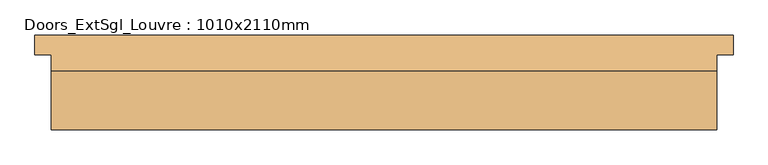
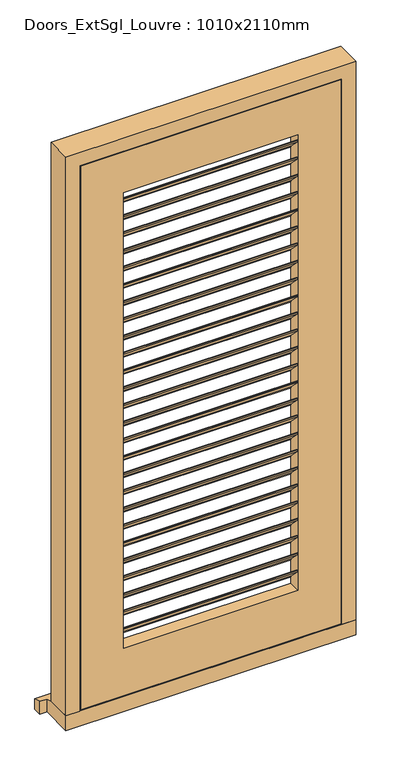
"""IFC4 building model written with IfcOpenShell, lengths in millimetres: door geometry, Doors_ExtSgl_Louvre : 1010x2110mm."""

from ifc_helpers import new_model, si_unit, point, frame, frame_2d, origin, place, context, project, spatial, polyline, circle_curve, trimmed, segment, composite_curve, outline, extrude, faceted_brep, source, transform, mapped, element, save


def doors_extsgl_louvre_1010x2110mm_50524d4c(model_context):
    return source(origin(), model_context, "Body", "SolidModel", [
        extrude(outline(composite_curve([segment(trimmed(circle_curve(frame_2d((1200.0, -378.5)), 19.0), [point((1200.0, -359.5))], [point((1200.0, -397.5))], False, "CARTESIAN"), True, "CONTINUOUS"), segment(trimmed(circle_curve(frame_2d((1200.0, -378.5)), 19.0), [point((1200.0, -397.5))], [point((1200.0, -359.5))], False, "CARTESIAN"), True, "CONTINUOUS")], self_intersect=False), holes=[composite_curve([segment(polyline([(1197.6985978, -377.5235023), (1188.3126735, -377.5235023), (1188.3126735, -379.4936963), (1197.7059713, -379.4936963)]), True, "CONTINUOUS"), segment(trimmed(circle_curve(frame_2d((1200.0, -378.5)), 2.5), [point((1197.7059713, -379.4936963))], [point((1197.6985978, -377.5235023))], True, "CARTESIAN"), True, "CONTINUOUS")], self_intersect=False)]), frame((0.0, 96.25, 0.0), z_axis=(0.0, 1.0, 0.0), x_axis=(0.0, 0.0, 1.0)), (0.0, 0.0, 1.0), 3.0),
        extrude(outline(polyline([(56.25, 1821.22), (96.25, 1781.22), (96.25, 1777.22), (93.25, 1777.22), (93.25, 1779.9773593), (53.25, 1819.9773593), (53.25, 1825.22), (56.25, 1825.22), (56.25, 1821.22)])), frame((-303.5, 0.0, 0.0), z_axis=(1.0, 0.0, 0.0), x_axis=(0.0, 1.0, 0.0)), (0.0, 0.0, 1.0), 607.0),
        extrude(outline(polyline([(56.25, 1757.94), (96.25, 1717.94), (96.25, 1713.94), (93.25, 1713.94), (93.25, 1716.6973593), (53.25, 1756.6973593), (53.25, 1761.94), (56.25, 1761.94), (56.25, 1757.94)])), frame((-303.5, 0.0, 0.0), z_axis=(1.0, 0.0, 0.0), x_axis=(0.0, 1.0, 0.0)), (0.0, 0.0, 1.0), 607.0),
        extrude(outline(polyline([(56.25, 1694.66), (96.25, 1654.66), (96.25, 1650.66), (93.25, 1650.66), (93.25, 1653.4173593), (53.25, 1693.4173593), (53.25, 1698.66), (56.25, 1698.66), (56.25, 1694.66)])), frame((-303.5, 0.0, 0.0), z_axis=(1.0, 0.0, 0.0), x_axis=(0.0, 1.0, 0.0)), (0.0, 0.0, 1.0), 607.0),
        extrude(outline(polyline([(56.25, 1631.38), (96.25, 1591.38), (96.25, 1587.38), (93.25, 1587.38), (93.25, 1590.1373593), (53.25, 1630.1373593), (53.25, 1635.38), (56.25, 1635.38), (56.25, 1631.38)])), frame((-303.5, 0.0, 0.0), z_axis=(1.0, 0.0, 0.0), x_axis=(0.0, 1.0, 0.0)), (0.0, 0.0, 1.0), 607.0),
        extrude(outline(polyline([(56.25, 1568.1), (96.25, 1528.1), (96.25, 1524.1), (93.25, 1524.1), (93.25, 1526.8573593), (53.25, 1566.8573593), (53.25, 1572.1), (56.25, 1572.1), (56.25, 1568.1)])), frame((-303.5, 0.0, 0.0), z_axis=(1.0, 0.0, 0.0), x_axis=(0.0, 1.0, 0.0)), (0.0, 0.0, 1.0), 607.0),
        extrude(outline(polyline([(56.25, 1504.82), (96.25, 1464.82), (96.25, 1460.82), (93.25, 1460.82), (93.25, 1463.5773593), (53.25, 1503.5773593), (53.25, 1508.82), (56.25, 1508.82), (56.25, 1504.82)])), frame((-303.5, 0.0, 0.0), z_axis=(1.0, 0.0, 0.0), x_axis=(0.0, 1.0, 0.0)), (0.0, 0.0, 1.0), 607.0),
        extrude(outline(polyline([(56.25, 1441.54), (96.25, 1401.54), (96.25, 1397.54), (93.25, 1397.54), (93.25, 1400.2973593), (53.25, 1440.2973593), (53.25, 1445.54), (56.25, 1445.54), (56.25, 1441.54)])), frame((-303.5, 0.0, 0.0), z_axis=(1.0, 0.0, 0.0), x_axis=(0.0, 1.0, 0.0)), (0.0, 0.0, 1.0), 607.0),
        extrude(outline(polyline([(56.25, 1378.26), (96.25, 1338.26), (96.25, 1334.26), (93.25, 1334.26), (93.25, 1337.0173593), (53.25, 1377.0173593), (53.25, 1382.26), (56.25, 1382.26), (56.25, 1378.26)])), frame((-303.5, 0.0, 0.0), z_axis=(1.0, 0.0, 0.0), x_axis=(0.0, 1.0, 0.0)), (0.0, 0.0, 1.0), 607.0),
        extrude(outline(polyline([(56.25, 1314.98), (96.25, 1274.98), (96.25, 1270.98), (93.25, 1270.98), (93.25, 1273.7373593), (53.25, 1313.7373593), (53.25, 1318.98), (56.25, 1318.98), (56.25, 1314.98)])), frame((-303.5, 0.0, 0.0), z_axis=(1.0, 0.0, 0.0), x_axis=(0.0, 1.0, 0.0)), (0.0, 0.0, 1.0), 607.0),
        extrude(outline(polyline([(56.25, 1251.7), (96.25, 1211.7), (96.25, 1207.7), (93.25, 1207.7), (93.25, 1210.4573593), (53.25, 1250.4573593), (53.25, 1255.7), (56.25, 1255.7), (56.25, 1251.7)])), frame((-303.5, 0.0, 0.0), z_axis=(1.0, 0.0, 0.0), x_axis=(0.0, 1.0, 0.0)), (0.0, 0.0, 1.0), 607.0),
        extrude(outline(polyline([(56.25, 1188.42), (96.25, 1148.42), (96.25, 1144.42), (93.25, 1144.42), (93.25, 1147.1773593), (53.25, 1187.1773593), (53.25, 1192.42), (56.25, 1192.42), (56.25, 1188.42)])), frame((-303.5, 0.0, 0.0), z_axis=(1.0, 0.0, 0.0), x_axis=(0.0, 1.0, 0.0)), (0.0, 0.0, 1.0), 607.0),
        extrude(outline(polyline([(56.25, 1125.14), (96.25, 1085.14), (96.25, 1081.14), (93.25, 1081.14), (93.25, 1083.8973593), (53.25, 1123.8973593), (53.25, 1129.14), (56.25, 1129.14), (56.25, 1125.14)])), frame((-303.5, 0.0, 0.0), z_axis=(1.0, 0.0, 0.0), x_axis=(0.0, 1.0, 0.0)), (0.0, 0.0, 1.0), 607.0),
        extrude(outline(polyline([(56.25, 1061.86), (96.25, 1021.86), (96.25, 1017.86), (93.25, 1017.86), (93.25, 1020.6173593), (53.25, 1060.6173593), (53.25, 1065.86), (56.25, 1065.86), (56.25, 1061.86)])), frame((-303.5, 0.0, 0.0), z_axis=(1.0, 0.0, 0.0), x_axis=(0.0, 1.0, 0.0)), (0.0, 0.0, 1.0), 607.0),
        extrude(outline(polyline([(56.25, 998.58), (96.25, 958.58), (96.25, 954.58), (93.25, 954.58), (93.25, 957.3373593), (53.25, 997.3373593), (53.25, 1002.58), (56.25, 1002.58), (56.25, 998.58)])), frame((-303.5, 0.0, 0.0), z_axis=(1.0, 0.0, 0.0), x_axis=(0.0, 1.0, 0.0)), (0.0, 0.0, 1.0), 607.0),
        extrude(outline(polyline([(56.25, 935.3), (96.25, 895.3), (96.25, 891.3), (93.25, 891.3), (93.25, 894.0573593), (53.25, 934.0573593), (53.25, 939.3), (56.25, 939.3), (56.25, 935.3)])), frame((-303.5, 0.0, 0.0), z_axis=(1.0, 0.0, 0.0), x_axis=(0.0, 1.0, 0.0)), (0.0, 0.0, 1.0), 607.0),
        extrude(outline(polyline([(56.25, 872.02), (96.25, 832.02), (96.25, 828.02), (93.25, 828.02), (93.25, 830.7773593), (53.25, 870.7773593), (53.25, 876.02), (56.25, 876.02), (56.25, 872.02)])), frame((-303.5, 0.0, 0.0), z_axis=(1.0, 0.0, 0.0), x_axis=(0.0, 1.0, 0.0)), (0.0, 0.0, 1.0), 607.0),
        extrude(outline(polyline([(56.25, 808.74), (96.25, 768.74), (96.25, 764.74), (93.25, 764.74), (93.25, 767.4973593), (53.25, 807.4973593), (53.25, 812.74), (56.25, 812.74), (56.25, 808.74)])), frame((-303.5, 0.0, 0.0), z_axis=(1.0, 0.0, 0.0), x_axis=(0.0, 1.0, 0.0)), (0.0, 0.0, 1.0), 607.0),
        extrude(outline(polyline([(56.25, 745.46), (96.25, 705.46), (96.25, 701.46), (93.25, 701.46), (93.25, 704.2173593), (53.25, 744.2173593), (53.25, 749.46), (56.25, 749.46), (56.25, 745.46)])), frame((-303.5, 0.0, 0.0), z_axis=(1.0, 0.0, 0.0), x_axis=(0.0, 1.0, 0.0)), (0.0, 0.0, 1.0), 607.0),
        extrude(outline(polyline([(56.25, 682.18), (96.25, 642.18), (96.25, 638.18), (93.25, 638.18), (93.25, 640.9373593), (53.25, 680.9373593), (53.25, 686.18), (56.25, 686.18), (56.25, 682.18)])), frame((-303.5, 0.0, 0.0), z_axis=(1.0, 0.0, 0.0), x_axis=(0.0, 1.0, 0.0)), (0.0, 0.0, 1.0), 607.0),
        extrude(outline(polyline([(56.25, 618.9), (96.25, 578.9), (96.25, 574.9), (93.25, 574.9), (93.25, 577.6573593), (53.25, 617.6573593), (53.25, 622.9), (56.25, 622.9), (56.25, 618.9)])), frame((-303.5, 0.0, 0.0), z_axis=(1.0, 0.0, 0.0), x_axis=(0.0, 1.0, 0.0)), (0.0, 0.0, 1.0), 607.0),
        extrude(outline(polyline([(56.25, 555.62), (96.25, 515.62), (96.25, 511.62), (93.25, 511.62), (93.25, 514.3773593), (53.25, 554.3773593), (53.25, 559.62), (56.25, 559.62), (56.25, 555.62)])), frame((-303.5, 0.0, 0.0), z_axis=(1.0, 0.0, 0.0), x_axis=(0.0, 1.0, 0.0)), (0.0, 0.0, 1.0), 607.0),
        extrude(outline(polyline([(56.25, 492.34), (96.25, 452.34), (96.25, 448.34), (93.25, 448.34), (93.25, 451.0973593), (53.25, 491.0973593), (53.25, 496.34), (56.25, 496.34), (56.25, 492.34)])), frame((-303.5, 0.0, 0.0), z_axis=(1.0, 0.0, 0.0), x_axis=(0.0, 1.0, 0.0)), (0.0, 0.0, 1.0), 607.0),
        extrude(outline(polyline([(56.25, 429.06), (96.25, 389.06), (96.25, 385.06), (93.25, 385.06), (93.25, 387.8173593), (53.25, 427.8173593), (53.25, 433.06), (56.25, 433.06), (56.25, 429.06)])), frame((-303.5, 0.0, 0.0), z_axis=(1.0, 0.0, 0.0), x_axis=(0.0, 1.0, 0.0)), (0.0, 0.0, 1.0), 607.0),
        extrude(outline(polyline([(56.25, 365.78), (96.25, 325.78), (96.25, 321.78), (93.25, 321.78), (93.25, 324.5373593), (53.25, 364.5373593), (53.25, 369.78), (56.25, 369.78), (56.25, 365.78)])), frame((-303.5, 0.0, 0.0), z_axis=(1.0, 0.0, 0.0), x_axis=(0.0, 1.0, 0.0)), (0.0, 0.0, 1.0), 607.0),
        extrude(outline(polyline([(56.25, 1884.5), (96.25, 1844.5), (96.25, 1840.5), (93.25, 1840.5), (93.25, 1843.2573593), (53.25, 1883.2573593), (53.25, 1888.5), (56.25, 1888.5), (56.25, 1884.5)])), frame((-303.5, 0.0, 0.0), z_axis=(1.0, 0.0, 0.0), x_axis=(0.0, 1.0, 0.0)), (0.0, 0.0, 1.0), 607.0),
        extrude(outline(polyline([(56.25, 302.5), (96.25, 262.5), (96.25, 258.5), (93.25, 258.5), (93.25, 261.2573593), (53.25, 301.2573593), (53.25, 306.5), (56.25, 306.5), (56.25, 302.5)])), frame((-303.5, 0.0, 0.0), z_axis=(1.0, 0.0, 0.0), x_axis=(0.0, 1.0, 0.0)), (0.0, 0.0, 1.0), 607.0),
        faceted_brep([(434.5, 141.25, 54.5), (505.0, 141.25, 54.5), (505.0, 52.25, 54.5), (456.5, 52.25, 54.5), (456.5, 99.25, 54.5), (434.5, 99.25, 54.5), (434.5, 141.25, 2039.5), (-434.5, 141.25, 2039.5), (-434.5, 141.25, 54.5), (-505.0, 141.25, 54.5), (-505.0, 141.25, 2110.0), (505.0, 141.25, 2110.0), (505.0, 52.25, 2110.0), (-505.0, 52.25, 2110.0), (-505.0, 52.25, 54.5), (-456.5, 52.25, 54.5), (-456.5, 52.25, 2061.5), (456.5, 52.25, 2061.5), (456.5, 99.25, 2061.5), (-456.5, 99.25, 2061.5), (-456.5, 99.25, 54.5), (-434.5, 99.25, 54.5), (-434.5, 99.25, 2039.5), (434.5, 99.25, 2039.5)], [[[0, 1, 2, 3, 4, 5]], [[1, 0, 6, 7, 8, 9, 10, 11]], [[2, 1, 11, 12]], [[3, 2, 12, 13, 14, 15, 16, 17]], [[4, 3, 17, 18]], [[5, 4, 18, 19, 20, 21, 22, 23]], [[0, 5, 23, 6]], [[7, 22, 21, 8]], [[8, 21, 20, 15, 14, 9]], [[13, 10, 9, 14]], [[19, 16, 15, 20]], [[12, 11, 10, 13]], [[18, 17, 16, 19]], [[6, 23, 22, 7]]]),
        faceted_brep([(530.0, 196.25, 0.0), (530.0, 196.25, 38.5947221), (530.0, 166.25, 47.2703282), (530.0, 166.25, 0.0), (-530.0, 196.25, 38.5947221), (-530.0, 196.25, 0.0), (-530.0, 166.25, 0.0), (-530.0, 166.25, 47.2703282), (505.0, 166.25, 0.0), (505.0, 52.25, 0.0), (-505.0, 52.25, 0.0), (-505.0, 166.25, 0.0), (-505.0, 166.25, 47.2703282), (-505.0, 141.25, 54.5), (505.0, 141.25, 54.5), (505.0, 166.25, 47.2703282), (-505.0, 52.25, 54.5), (505.0, 52.25, 54.5)], [[[0, 1, 2, 3]], [[4, 5, 6, 7]], [[5, 0, 3, 8, 9, 10, 11, 6]], [[1, 0, 5, 4]], [[1, 4, 7, 12, 13, 14, 15, 2]], [[13, 16, 17, 14]], [[16, 10, 9, 17]], [[12, 11, 10, 16, 13]], [[11, 12, 7, 6]], [[8, 15, 14, 17, 9]], [[15, 8, 3, 2]]]),
        extrude(outline(polyline([(58.5, 453.5), (2058.5, 453.5), (2058.5, -454.4250294), (58.5, -454.4250294), (58.5, 453.5)]), holes=[polyline([(233.5, -303.5), (1908.5, -303.5), (1908.5, 303.5), (233.5, 303.5), (233.5, -303.5)])]), frame((0.0, 52.25, 0.0), z_axis=(0.0, 1.0, 0.0), x_axis=(0.0, 0.0, 1.0)), (0.0, 0.0, 1.0), 44.0),
    ])


if __name__ == "__main__":
    model = new_model("IFC4")
    model_context = context("Model", 3, world=origin())
    ifc_project = project(units=[si_unit("LENGTHUNIT", "METRE", prefix="MILLI")], contexts=[model_context])
    site = spatial("IfcSite", under=ifc_project)
    building = spatial("IfcBuilding", under=site)
    placement = place(None, origin())
    doors_extsgl_louvre_1010x2110mm_shape = doors_extsgl_louvre_1010x2110mm_50524d4c(model_context)
    element("IfcDoor", 1, ObjectType="Doors_ExtSgl_Louvre : 1010x2110mm", at=placement, inside=building, context=model_context, shape_type="MappedRepresentation", body=[
        mapped(doors_extsgl_louvre_1010x2110mm_shape, transform((0.0, 0.0, 0.0), x_axis=(1.0, 0.0, 0.0), y_axis=(0.0, 1.0, 0.0), z_axis=(0.0, 0.0, 1.0))),
    ])
    save(model, "model.ifc")

# Revit data of these elements
# Type "Doors_ExtSgl_Louvre : 1010x2110mm"
#   Type Mark = "76"
#   Type Comments = "External Single"
#   Operation = "SingleSwingRight"
#   Construction Type Id = "MDOOR"
#   Keynote = "L20"
#   Analytic Construction = "Metal"
#   Wrap Layers (Int) from Ext = 177.5 mm
#   Wrap Layers (Ext) from Ext = 102.5 mm
#   Thickness = 44 mm
#   Stile Top Rail = 150 mm
#   Stile Shutting = 150 mm
#   Stile Hanging = 150 mm
#   Stile Bottom Rail = 175 mm
#   Rough Width = 1010 mm
#   Rough Height = 2110 mm
#   O/A Frame Width = 64 mm
#   Heat Transfer Coefficient (U) = 3.7021 W/(m²·K)
#   Handle Z Offset = 1200 mm
#   Handle X Offset = 75 mm
#   Glazing Thickness = 24 mm
#   FrameWidth = 42 mm
#   FrameOffset - External = 25 mm
#   FrameDepth = 89 mm
#   Door Panel Width = 907 mm
#   Door Panel Thickness = 44 mm
#   Door Panel Height = 2000 mm
#   DONT CHANGE Louvre Length = 607 mm
#   Cill Thickness = 54.5 mm
#   Cill Projection = 30 mm
#   Height = 2110 mm
#   Structural Tolerance = 6.5 mm
#   Tolerance = 3 mm
#   Undercut = 4 mm
#   Width = 1010 mm
#   Cill Extension = 25 mm
#   Cavity Closer Width = 50 mm
#   Cavity Closer Offset from Ext = 102.5 mm
#   Cavity Closer Depth = 85 mm
#   Vis - Ironmongery = yes
#   Vis - Cavity Closers = yes
#   Define Thermal Properties by = 1
#   No of Louvres = 26
#   Function = 1
#   Material Door = Door - Panel
#   Material Frame = Door - Frame/Mullion
#   Material Ironmongery = Door - Handle
#   Visual Light Transmittance = 0
#   Solar Heat Gain Coefficient = 0
#   Wall Closure = (empty or 0)
# Element 1 (IfcDoor, "Doors_ExtSgl_Louvre : 1010x2110mm")
#   Materials on its faces: "Door - Panel", "Door - Frame/Mullion", "Door - Handle"
# Materials
#   "Door - Panel": class "Wood", colour RGB 210 159 95, transparency 0, Keynote = "L20"
#   "Door - Frame/Mullion": class "Wood", colour RGB 212 179 113, transparency 0, Keynote = "L20"
#   "Door - Handle": class "Miscellaneous", colour RGB 0 0 0, transparency 0, Keynote = "P21"
